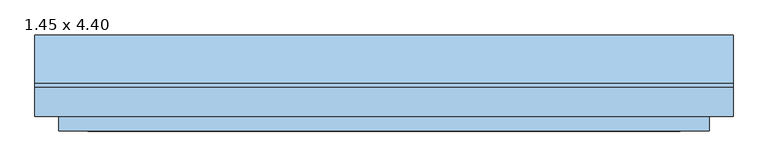
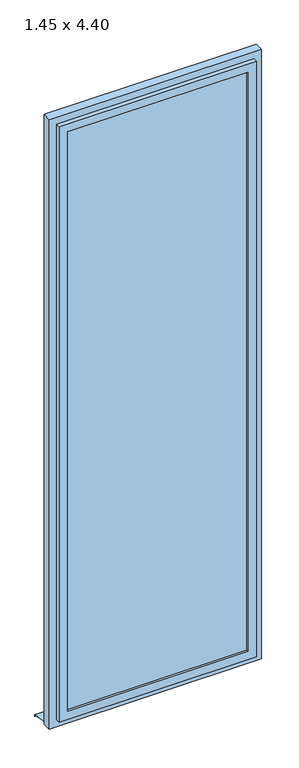
"""IFC4 building model written with IfcOpenShell, lengths in millimetres: window geometry, Fenstertür 1-flg : 1.45 x 4.40."""

from ifc_helpers import new_model, si_unit, frame, origin, place, context, project, spatial, polyline, outline, extrude, faceted_brep, source, transform, mapped, element, save


def window_1_45_x_4_40_0b14fd1c(model_context):
    return source(origin(), model_context, "Body", "SolidModel", [
        extrude(outline(polyline([(4400.0, 725.0), (4400.0, -725.0), (0.0, -725.0), (0.0, 725.0), (4400.0, 725.0)]), holes=[polyline([(4320.0, 645.0), (80.0, 645.0), (80.0, -645.0), (4320.0, -645.0), (4320.0, 645.0)])]), frame((0.0, 35.0, 0.0), z_axis=(0.0, 1.0, 0.0), x_axis=(0.0, 0.0, 1.0)), (0.0, 0.0, 1.0), 60.0),
        faceted_brep([(675.0, 35.0, 4350.0), (675.0, 5.0, 4350.0), (675.0, 5.0, 50.0), (675.0, 35.0, 50.0), (-675.0, 5.0, 4350.0), (-675.0, 5.0, 50.0), (615.0, 5.0, 110.0), (-615.0, 5.0, 110.0), (-615.0, 5.0, 4290.0), (615.0, 5.0, 4290.0), (-675.0, 35.0, 50.0), (-675.0, 35.0, 4350.0), (645.0, 35.0, 4320.0), (-645.0, 35.0, 4320.0), (-645.0, 35.0, 80.0), (645.0, 35.0, 80.0), (645.0, 65.0, 4320.0), (645.0, 65.0, 80.0), (-645.0, 65.0, 80.0), (-645.0, 65.0, 4320.0), (615.0, 65.0, 4290.0), (-615.0, 65.0, 4290.0), (-615.0, 65.0, 110.0), (615.0, 65.0, 110.0)], [[[0, 1, 2, 3]], [[1, 4, 5, 2], [6, 7, 8, 9]], [[3, 2, 5, 10]], [[3, 10, 11, 0], [12, 13, 14, 15]], [[16, 12, 15, 17]], [[17, 15, 14, 18]], [[17, 18, 19, 16], [20, 21, 22, 23]], [[9, 20, 23, 6]], [[6, 23, 22, 7]], [[10, 5, 4, 11]], [[18, 14, 13, 19]], [[7, 22, 21, 8]], [[11, 4, 1, 0]], [[19, 13, 12, 16]], [[8, 21, 20, 9]]]),
        extrude(outline(polyline([(105.0221543, 20.0), (205.0, 0.0), (205.0, -10.0), (203.0, -10.0), (203.0, -1.6395366), (104.8240723, 18.0), (95.0, 18.0), (95.0, 20.0), (105.0221543, 20.0)])), frame((-725.0, 0.0, 0.0), z_axis=(1.0, 0.0, 0.0), x_axis=(0.0, 1.0, 0.0)), (0.0, 0.0, 1.0), 1450.0),
        extrude(outline(polyline([(615.0, 20.0), (-615.0, 20.0), (-615.0, 50.0), (615.0, 50.0), (615.0, 20.0)])), frame((0.0, 0.0, 110.0), z_axis=(0.0, 0.0, 1.0), x_axis=(1.0, 0.0, 0.0)), (0.0, 0.0, 1.0), 4180.0),
    ])


if __name__ == "__main__":
    model = new_model("IFC4")
    model_context = context("Model", 3, world=origin())
    ifc_project = project(units=[si_unit("LENGTHUNIT", "METRE", prefix="MILLI")], contexts=[model_context])
    site = spatial("IfcSite", under=ifc_project)
    building = spatial("IfcBuilding", under=site)
    placement = place(None, origin())
    window_1_45_x_4_40_shape = window_1_45_x_4_40_0b14fd1c(model_context)
    element("IfcWindow", 1, ObjectType="Fenstertür 1-flg : 1.45 x 4.40", at=placement, inside=building, context=model_context, shape_type="MappedRepresentation", body=[
        mapped(window_1_45_x_4_40_shape, transform((0.0, 0.0, 0.0), x_axis=(1.0, 0.0, 0.0), y_axis=(0.0, 1.0, 0.0), z_axis=(0.0, 0.0, 1.0))),
    ])
    save(model, "model.ifc")

# Revit data of these elements
# Type "Fenstertür 1-flg : 1.45 x 4.40"
#   Type Mark = "57"
#   Operation = "SinglePanel"
#   Construction Type Id = "GSP4R"
#   Keynote = "16.05.01"
#   Analytic Construction = "1/8 Zoll Pilkington-Verglasung einfach"
#   Visual Light Transmittance = 0.9
#   Thermal Resistance (R) = 0.1491 (m²·K)/W
#   Solar Heat Gain Coefficient = 0.86
#   Rough Width = 1.450 m
#   Rough Height = 4.400 m
#   Heat Transfer Coefficient (U) = 6.7069 W/(m²·K)
#   Rahmentiefe = 0.060 m
#   Rahmenhöhe - unten = 0.080 m
#   Rahmenhöhe - oben = 0.080 m
#   Rahmenbreite = 0.080 m
#   Height = 4.400 m
#   Tiefe Flügel = 0.060 m
#   Flügelbreite = 0.060 m
#   Einbautiefe (von außen) [instance default] = 0.080 m
#   Width = 1.450 m
#   Kippflügel [instance default] = yes
#   Drehflügel im Grundriss darstellen [instance default] = yes
#   Drehflügel 1 [instance default] = yes
#   Rahmen 1 [instance default] = none
#   Glas [instance default] = none
#   Flügel [instance default] = none
#   Fensterbank Außenseite [instance default] = none
#   Wall Closure = (empty or 0)
# Element 1 (IfcWindow, "Fenstertür 1-flg : 1.45 x 4.40")
#   Materials on its faces: "Kunststoff - Weiß", "Glas"
# Materials
#   "Kunststoff - Weiß": class "Kunststoff", colour RGB 249 249 249, transparency 0, Cost = 0
#   "Glas": class "Glas", colour RGB 0 0 255, transparency 0.75, Comments = "Render-Darstellung nicht aktualisiert ", Cost = 0
